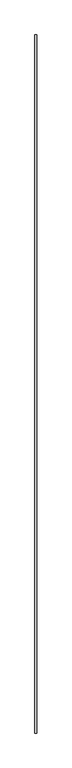
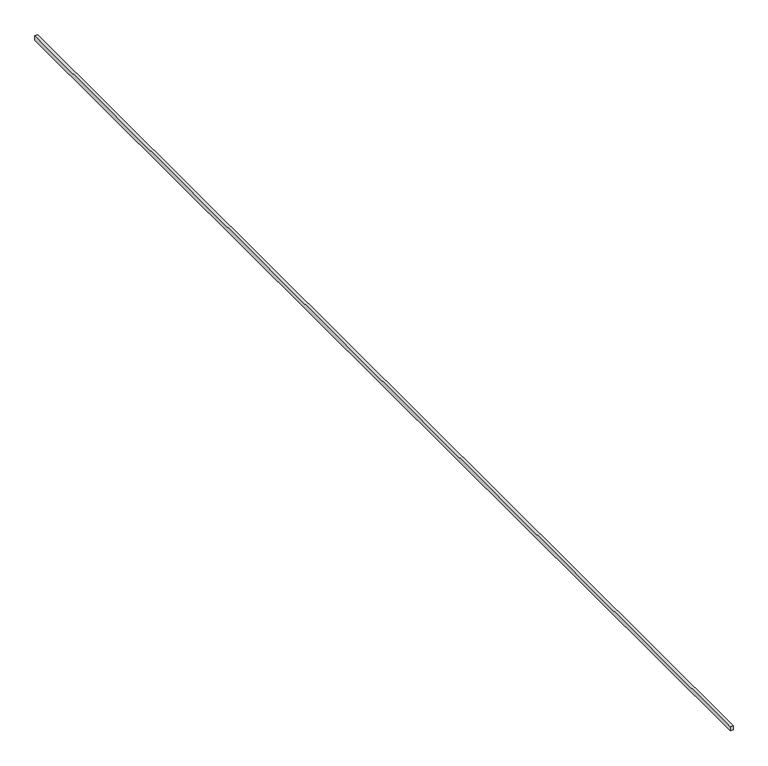
"""IFC4 building model written with IfcOpenShell, lengths in millimetres: proxy geometry, Generic Models 7:Generic Models 1:5:Generic Models 1:5 : Generic Models 7:Generic Models 1:337419:23 : Generic Models 7:Generic Models 1:5:Generic Models 1:5 : Generic Models 7:Generic Models 1:337419:311462."""

import ifcopenshell
import ifcopenshell.guid

model = None  # the IFC model being written
_history = None  # IfcOwnerHistory: only IFC2X3 demands one
_inside = {}  # id of a spatial element -> (the spatial element, [elements in it])
_under = {}  # id of a project, library or spatial element -> (it, [spatial elements below it])
_declared = {}  # id of a project -> (the project, [libraries it declares])
_typed = {}  # id of a type object -> (the type object, [elements of that type])
_made_of = {}  # id of a material, layer set ... -> (it, [elements and type objects made of it])


def new_model(schema):
    """Start an empty IFC model of exactly this schema.

    Asked for "IFC4X3", IfcOpenShell would pick the latest addendum, in which some entities
    have other attributes; the version numbers below select the first issue.
    IFC2X3 requires an IfcOwnerHistory on every rooted entity: one is made here for all.
    """
    global model, _history
    if schema == "IFC4X3":
        model = ifcopenshell.file(schema_version=(4, 3, 0, 0))
    else:
        model = ifcopenshell.file(schema=schema)
    _inside.clear()
    _under.clear()
    _declared.clear()
    _typed.clear()
    _made_of.clear()
    _history = None
    if model.schema == "IFC2X3":
        org = make("IfcOrganization", Name="unknown")
        user = make(
            "IfcPersonAndOrganization",
            ThePerson=make("IfcPerson", FamilyName="unknown"),
            TheOrganization=org,
        )
        app = make(
            "IfcApplication",
            ApplicationDeveloper=org,
            Version="unknown",
            ApplicationFullName="unknown",
            ApplicationIdentifier="unknown",
        )
        _history = make(
            "IfcOwnerHistory",
            OwningUser=user,
            OwningApplication=app,
            ChangeAction="ADDED",
            CreationDate=0,
        )
    return model


def make(cls, **values):
    """One entity of the class cls with the attributes given. An attribute that is None is left unset."""
    return model.create_entity(
        cls, **{name: value for name, value in values.items() if value is not None}
    )


def rooted(cls, **values):
    """An entity with a GlobalId (a new one), such as an element, a storey or a relation."""
    return make(cls, GlobalId=ifcopenshell.guid.new(), OwnerHistory=_history, **values)


def si_unit(unit_type, name, prefix=None):
    """IfcSIUnit, for example si_unit("LENGTHUNIT", "METRE", prefix="MILLI")."""
    return make("IfcSIUnit", UnitType=unit_type, Prefix=prefix, Name=name)


def assignment(units):
    """IfcUnitAssignment: the units of a project."""
    return None if units is None else make("IfcUnitAssignment", Units=units)


def point(xyz):
    """IfcCartesianPoint."""
    return None if xyz is None else make("IfcCartesianPoint", Coordinates=xyz)


def direction(xyz):
    """IfcDirection."""
    return None if xyz is None else make("IfcDirection", DirectionRatios=xyz)


def frame(location, z_axis=None, x_axis=None):
    """IfcAxis2Placement3D, a coordinate frame: its origin and axes. An axis left out is left unset."""
    return make(
        "IfcAxis2Placement3D",
        Location=point(location),
        Axis=direction(z_axis),
        RefDirection=direction(x_axis),
    )


def origin():
    """The frame at (0, 0, 0) with its axes left unset."""
    return frame((0.0, 0.0, 0.0))


def place(relative_to, where):
    """IfcLocalPlacement: puts the frame where relative to a parent placement (None: the world)."""
    return make(
        "IfcLocalPlacement", PlacementRelTo=relative_to, RelativePlacement=where
    )


def context(
    kind, dimensions, precision=None, world=None, true_north=None, identifier=None
):
    """IfcGeometricRepresentationContext, for example the 3D "Model" context."""
    return make(
        "IfcGeometricRepresentationContext",
        ContextIdentifier=identifier,
        ContextType=kind,
        CoordinateSpaceDimension=dimensions,
        Precision=precision,
        WorldCoordinateSystem=world,
        TrueNorth=true_north,
    )


def project(units=None, contexts=None):
    """IfcProject with its units and contexts."""
    return rooted(
        "IfcProject",
        Name="project",
        RepresentationContexts=contexts,
        UnitsInContext=assignment(units),
    )


def spatial(cls, under=None, at=None, **own):
    """A site, building, storey or space (cls), placed at a placement, below another one or the project."""
    s = rooted(cls, ObjectPlacement=at, **own)
    if under is not None:
        _under.setdefault(under.id(), (under, []))[1].append(s)
    return s


def polyline(points):
    """IfcPolyline through the points."""
    return make("IfcPolyline", Points=[point(p) for p in points])


def outline(outer, holes=None, kind="AREA"):
    """IfcArbitraryClosedProfileDef: a profile drawn as a closed curve; with holes, ...WithVoids."""
    if holes is None:
        return make("IfcArbitraryClosedProfileDef", ProfileType=kind, OuterCurve=outer)
    return make(
        "IfcArbitraryProfileDefWithVoids",
        ProfileType=kind,
        OuterCurve=outer,
        InnerCurves=holes,
    )


def extrude(swept, where, along, depth):
    """IfcExtrudedAreaSolid: the profile swept, set in the frame where, extruded along a direction by depth."""
    return make(
        "IfcExtrudedAreaSolid",
        SweptArea=swept,
        Position=where,
        ExtrudedDirection=direction(along),
        Depth=depth,
    )


def shape(context_of_items, identifier, shape_type, items):
    """IfcShapeRepresentation: the items that make up one representation, for example the "Body"."""
    return make(
        "IfcShapeRepresentation",
        ContextOfItems=context_of_items,
        RepresentationIdentifier=identifier,
        RepresentationType=shape_type,
        Items=items,
    )


def source(mapping_origin, context_of_items, identifier, shape_type, items):
    """IfcRepresentationMap: a shape defined once, which mapped items show again and again."""
    return make(
        "IfcRepresentationMap",
        MappingOrigin=mapping_origin,
        MappedRepresentation=shape(context_of_items, identifier, shape_type, items),
    )


def transform(
    local_origin,
    x_axis=None,
    y_axis=None,
    z_axis=None,
    scale=None,
    scale2=None,
    scale3=None,
    uniform=True,
):
    """IfcCartesianTransformationOperator3D, or its non-uniform kind. x_axis, y_axis, z_axis: its Axis1, 2, 3."""
    if uniform:
        return make(
            "IfcCartesianTransformationOperator3D",
            Axis1=direction(x_axis),
            Axis2=direction(y_axis),
            LocalOrigin=point(local_origin),
            Scale=scale,
            Axis3=direction(z_axis),
        )
    return make(
        "IfcCartesianTransformationOperator3DnonUniform",
        Axis1=direction(x_axis),
        Axis2=direction(y_axis),
        LocalOrigin=point(local_origin),
        Scale=scale,
        Axis3=direction(z_axis),
        Scale2=scale2,
        Scale3=scale3,
    )


def mapped(mapping_source, mapping_target):
    """IfcMappedItem: shows the shape of a source again, moved by a transform."""
    return make(
        "IfcMappedItem", MappingSource=mapping_source, MappingTarget=mapping_target
    )


def made_of(thing, what):
    """Note that an element or type object is made of a material, layer set ...; save() writes the relation."""
    if what is not None:
        _made_of.setdefault(what.id(), (what, []))[1].append(thing)
    return thing


def element(
    cls,
    number,
    at=None,
    inside=None,
    cuts=None,
    type_object=None,
    material=None,
    context=None,
    identifier="Body",
    shape_type=None,
    held_by="IfcProductDefinitionShape",
    body=None,
    shapes=None,
    **own,
):
    """One element of the class cls, such as IfcWall. Its Tag is "e" and its number.

    at: its placement. inside: the storey or other place that contains it. cuts: it is an
    opening in that element (IfcRelVoidsElement). A single representation is given by context,
    identifier, shape_type and body (its items); several are given by shapes. held_by: the class
    of the entity that holds the representations. save() writes the other relations.
    """
    e = rooted(cls, Tag="e%d" % number, ObjectPlacement=at, **own)
    if body is not None:
        shapes = [shape(context, identifier, shape_type, body)]
    if shapes is not None:
        e.Representation = make(held_by, Representations=shapes)
    if inside is not None:
        _inside.setdefault(inside.id(), (inside, []))[1].append(e)
    if cuts is not None:
        rooted(
            "IfcRelVoidsElement", RelatingBuildingElement=cuts, RelatedOpeningElement=e
        )
    if type_object is not None:
        _typed.setdefault(type_object.id(), (type_object, []))[1].append(e)
    return made_of(e, material)


def aggregate(whole, parts):
    """IfcRelAggregates: a whole, such as a stair, and the parts it consists of."""
    return rooted("IfcRelAggregates", RelatingObject=whole, RelatedObjects=parts)


def save(model, path):
    """Write the relations noted so far, then the file.

    IfcRelAggregates (storeys below a building ...), IfcRelContainedInSpatialStructure (elements
    in a storey), IfcRelDefinesByType, IfcRelAssociatesMaterial and IfcRelDeclares: one each for
    every whole, place, type object, material and project.
    """
    for whole, parts in _under.values():
        aggregate(whole, parts)
    for where, things in _inside.values():
        rooted(
            "IfcRelContainedInSpatialStructure",
            RelatedElements=things,
            RelatingStructure=where,
        )
    for kind, things in _typed.values():
        rooted("IfcRelDefinesByType", RelatedObjects=things, RelatingType=kind)
    for what, things in _made_of.values():
        rooted("IfcRelAssociatesMaterial", RelatedObjects=things, RelatingMaterial=what)
    for by, libraries in _declared.values():
        rooted("IfcRelDeclares", RelatingContext=by, RelatedDefinitions=libraries)
    model.write(path)


def generic_models_ba025cea(model_context):
    return source(origin(), model_context, "Body", "SweptSolid", [
        extrude(outline(polyline([(578647.3117239, -568215.2163841), (578621.8863239, -568215.2163841), (578621.8863239, -558080.616384), (578647.3117239, -558080.616384), (578647.3117239, -568215.2163841)])), frame((0.0, 0.0, 4876.8), z_axis=(0.0, 0.0, 1.0), x_axis=(1.0, 0.0, 0.0)), (0.0, 0.0, 1.0), 38.6419652),
    ])


if __name__ == "__main__":
    model = new_model("IFC4")
    model_context = context("Model", 3, world=origin())
    ifc_project = project(units=[si_unit("LENGTHUNIT", "METRE", prefix="MILLI")], contexts=[model_context])
    site = spatial("IfcSite", under=ifc_project)
    building = spatial("IfcBuilding", under=site)
    placement = place(None, origin())
    generic_models_shape = generic_models_ba025cea(model_context)
    element("IfcBuildingElementProxy", 1, Name="Generic Models 7:Generic Models 1:5:Generic Models 1:5 : Generic Models 7:Generic Models 1:337419:23 : Generic Models 7:Generic Models 1:5:Generic Models 1:5 : Generic Models 7:Generic Models 1:337419:311462", ObjectType="Generic Models 7:Generic Models 1:5:Generic Models 1:5 : Generic Models 7:Generic Models 1:337419:23 : Generic Models 7:Generic Models 1:5:Generic Models 1:5 : Generic Models 7:Generic Models 1:337419:311462", at=placement, inside=building, context=model_context, shape_type="MappedRepresentation", body=[
        mapped(generic_models_shape, transform((0.0, 0.0, 0.0), x_axis=(1.0, 0.0, 0.0), y_axis=(0.0, 1.0, 0.0), z_axis=(0.0, 0.0, 1.0))),
    ])
    save(model, "model.ifc")

# Revit data of these elements
# Type "Generic Models 7:Generic Models 1:5:Generic Models 1:5 : Generic Models 7:Generic Models 1:337419:23 : Generic Models 7:Generic Models 1:5:Generic Models 1:5 : Generic Models 7:Generic Models 1:337419:311462"
#   NameOverride = "Generic Models 7:Generic Models 1:5:Generic Models 1:5 : Generic Models 7:Generic Models 1:337419:311462"
#   ObjectTypeOverride = "Generic Models 1:5 : Generic Models 7:Generic Models 1:337419"
#   Reference = "Generic Models 1"
#   Tag = "311462"
# Element 1 (IfcBuildingElementProxy, "Generic Models 7:Generic Models 1:5:Generic Models 1:5 : Generic Models 7:Generic Models 1:337419:23 : Generic Models 7:Generic Models 1:5:Generic Models 1:5 : Generic Models 7:Generic Models 1:337419:311462")
#   Materials on its faces: "1\" THERMAL SPACER @ GIRT"
# Materials
#   "1\" THERMAL SPACER @ GIRT": class "Unassigned", colour RGB 205 188 106, transparency 0, Cost = 0
